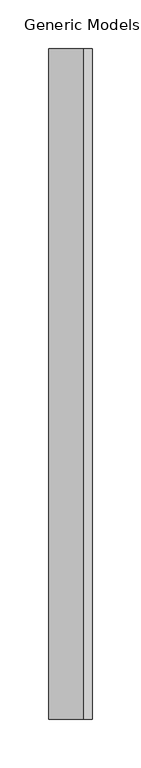
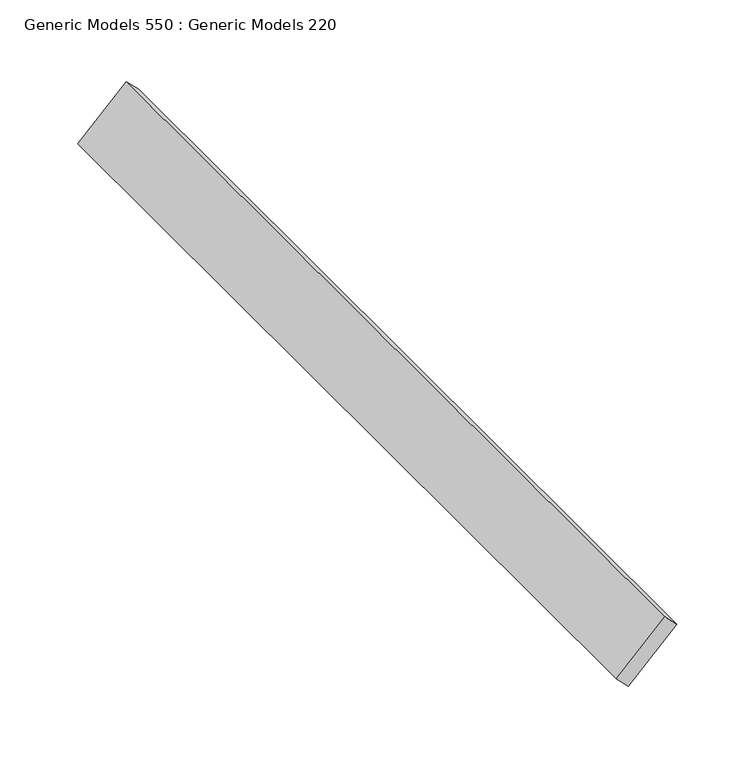
"""IFC4 building model written with IfcOpenShell, lengths in millimetres: proxy geometry, Generic Models 550 : Generic Models 220."""

from ifc_helpers import new_model, si_unit, frame, origin, place, context, project, spatial, polyline, outline, extrude, source, transform, mapped, element, save


def generic_models_550_generic_models_220_00ddf798(model_context):
    return source(origin(), model_context, "Body", "SweptSolid", [
        extrude(outline(polyline([(0.0, -12.7000001), (0.0, 0.0), (690.8142348, 0.0), (690.8142348, -12.7000001), (0.0, -12.7000001)])), frame((7841.3059863, 4539.4872686, 124684.1399101), z_axis=(0.7071067811868034, 0.0, 0.7071067811862918), x_axis=(0.0, -1.0, 0.0)), (0.0, 0.0, 1.0), 50.8),
    ])


if __name__ == "__main__":
    model = new_model("IFC4")
    model_context = context("Model", 3, world=origin())
    ifc_project = project(units=[si_unit("LENGTHUNIT", "METRE", prefix="MILLI")], contexts=[model_context])
    site = spatial("IfcSite", under=ifc_project)
    building = spatial("IfcBuilding", under=site)
    placement = place(None, origin())
    generic_models_550_generic_models_220_shape = generic_models_550_generic_models_220_00ddf798(model_context)
    element("IfcBuildingElementProxy", 1, Name="Generic Models 550 : Generic Models 220", ObjectType="Generic Models 550 : Generic Models 220", at=placement, inside=building, context=model_context, shape_type="MappedRepresentation", body=[
        mapped(generic_models_550_generic_models_220_shape, transform((0.0, 0.0, 0.0), x_axis=(1.0, 0.0, 0.0), y_axis=(0.0, 1.0, 0.0), z_axis=(0.0, 0.0, 1.0))),
    ])
    save(model, "model.ifc")

# Revit data of these elements
# Project information
#   Project Issue Date = "Issue Date"
#   Project Status = "Project Status"
#   Client Name = "Owner"
#   Project Address = "Enter address here"
#   Project Name = "Project Name"
#   Project Number = "Project Number"
# Element 1 (IfcBuildingElementProxy, "Generic Models 550 : Generic Models 220")
#   Materials on its faces: "_WOOD TONE ALUMINUM EXTRUSION SLAT BY KNOTWOOD"
# Materials
#   "_WOOD TONE ALUMINUM EXTRUSION SLAT BY KNOTWOOD": class "Generic", colour RGB 177 130 114, transparency 0, Cost = 0
